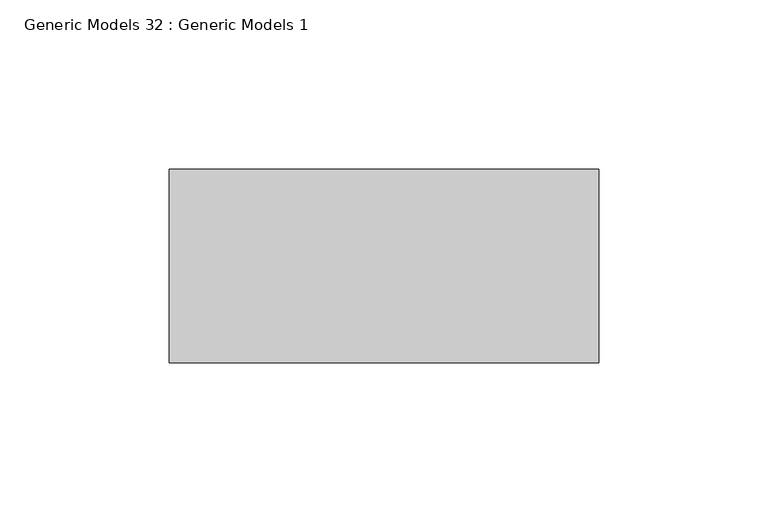
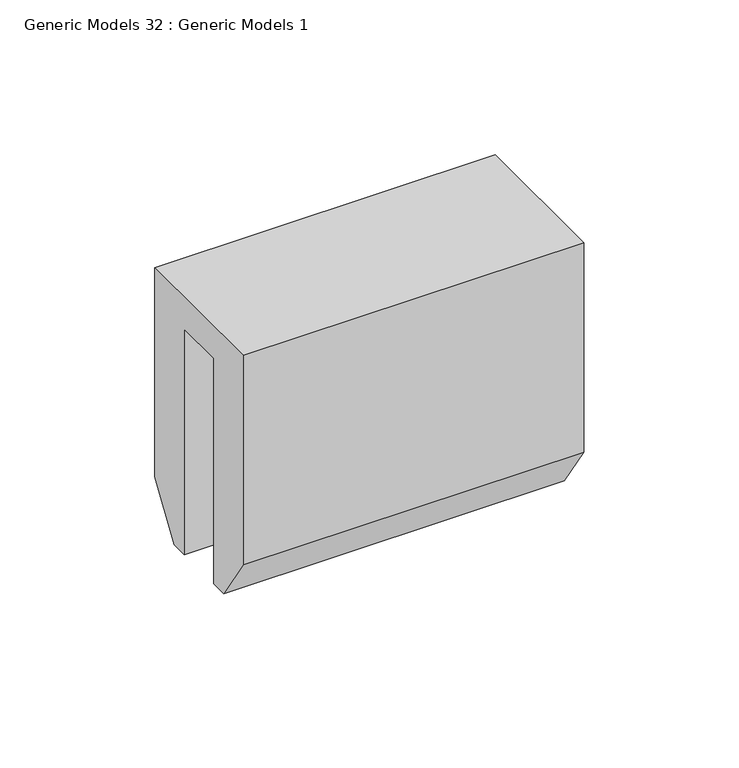
"""IFC4 building model written with IfcOpenShell, lengths in millimetres: proxy geometry, Generic Models 32 : Generic Models 1."""

from ifc_helpers import new_model, si_unit, frame, origin, place, context, project, spatial, polyline, outline, extrude, source, transform, mapped, element, save


def generic_models_32_generic_models_1_73908315(model_context):
    return source(origin(), model_context, "Body", "SweptSolid", [
        extrude(outline(polyline([(5685.0969995, 2889.1860265), (5685.0969995, 2806.6360265), (5672.3969995, 2787.5860265), (5666.0469995, 2787.5860265), (5666.0469995, 2876.4860265), (5646.9969995, 2876.4860265), (5646.9969995, 2787.5860265), (5640.6469995, 2787.5860265), (5627.9469995, 2806.6360265), (5627.9469995, 2889.1860265), (5685.0969995, 2889.1860265)])), frame((13805.7842846, 0.0, 0.0), z_axis=(1.0, 0.0, 0.0), x_axis=(0.0, 1.0, 0.0)), (0.0, 0.0, 1.0), 127.0),
    ])


if __name__ == "__main__":
    model = new_model("IFC4")
    model_context = context("Model", 3, world=origin())
    ifc_project = project(units=[si_unit("LENGTHUNIT", "METRE", prefix="MILLI")], contexts=[model_context])
    site = spatial("IfcSite", under=ifc_project)
    building = spatial("IfcBuilding", under=site)
    placement = place(None, origin())
    generic_models_32_generic_models_1_shape = generic_models_32_generic_models_1_73908315(model_context)
    element("IfcBuildingElementProxy", 1, Name="Generic Models 32 : Generic Models 1", ObjectType="Generic Models 32 : Generic Models 1", at=placement, inside=building, context=model_context, shape_type="MappedRepresentation", body=[
        mapped(generic_models_32_generic_models_1_shape, transform((0.0, 0.0, 0.0), x_axis=(1.0, 0.0, 0.0), y_axis=(0.0, 1.0, 0.0), z_axis=(0.0, 0.0, 1.0))),
    ])
    save(model, "model.ifc")

# Revit data of these elements
# Element 1 (IfcBuildingElementProxy, "Generic Models 32 : Generic Models 1")
#   Materials on its faces: "S.S.PATCH FITTING AT HINGE"
# Materials
#   "S.S.PATCH FITTING AT HINGE": class "Unassigned", colour RGB 210 209 208, transparency 0, Keynote = "M05121300.02", Cost = 0
